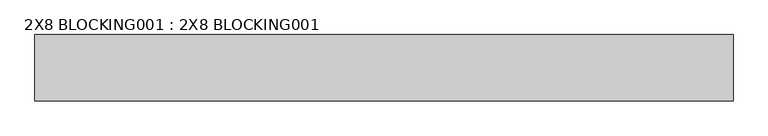
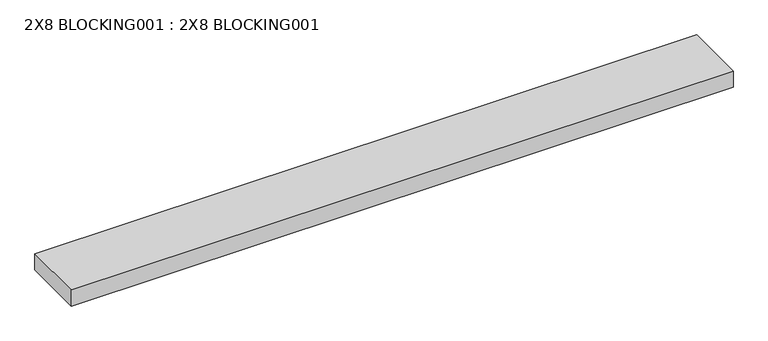
"""IFC4 building model written with IfcOpenShell, lengths in millimetres: proxy geometry, 2X8 BLOCKING001 : 2X8 BLOCKING001."""

from ifc_helpers import new_model, si_unit, frame, origin, place, context, project, spatial, polyline, outline, extrude, source, transform, mapped, element, save


def proxy_2x8_blocking001_2x8_blocking001_6d7b9a3e(model_context):
    return source(origin(), model_context, "Body", "SweptSolid", [
        extrude(outline(polyline([(12382.7678845, -5536.0675368), (12382.7678845, -5345.4245733), (14383.0178845, -5345.4245733), (14383.0178845, -5536.0675368), (12382.7678845, -5536.0675368)])), frame((0.0, 0.0, 40114.8623973), z_axis=(0.0, 0.0, 1.0), x_axis=(1.0, 0.0, 0.0)), (0.0, 0.0, 1.0), 51.9935355),
    ])


if __name__ == "__main__":
    model = new_model("IFC4")
    model_context = context("Model", 3, world=origin())
    ifc_project = project(units=[si_unit("LENGTHUNIT", "METRE", prefix="MILLI")], contexts=[model_context])
    site = spatial("IfcSite", under=ifc_project)
    building = spatial("IfcBuilding", under=site)
    placement = place(None, origin())
    proxy_2x8_blocking001_2x8_blocking001_shape = proxy_2x8_blocking001_2x8_blocking001_6d7b9a3e(model_context)
    element("IfcBuildingElementProxy", 1, Name="2X8 BLOCKING001 : 2X8 BLOCKING001", ObjectType="2X8 BLOCKING001 : 2X8 BLOCKING001", at=placement, inside=building, context=model_context, shape_type="MappedRepresentation", body=[
        mapped(proxy_2x8_blocking001_2x8_blocking001_shape, transform((0.0, 0.0, 0.0), x_axis=(1.0, 0.0, 0.0), y_axis=(0.0, 1.0, 0.0), z_axis=(0.0, 0.0, 1.0))),
    ])
    save(model, "model.ifc")

# Revit data of these elements
# Type "2X8 BLOCKING001 : 2X8 BLOCKING001"
#   NameOverride = "2X8 BLOCKING001"
# Element 1 (IfcBuildingElementProxy, "2X8 BLOCKING001 : 2X8 BLOCKING001")
#   Materials on its faces: "WOOD BLOCKING AS REQUIRED"
# Materials
#   "WOOD BLOCKING AS REQUIRED": class "Unassigned", colour RGB 166 124 85, transparency 0, Cost = 0
